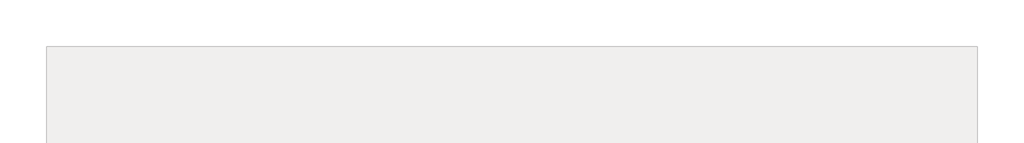
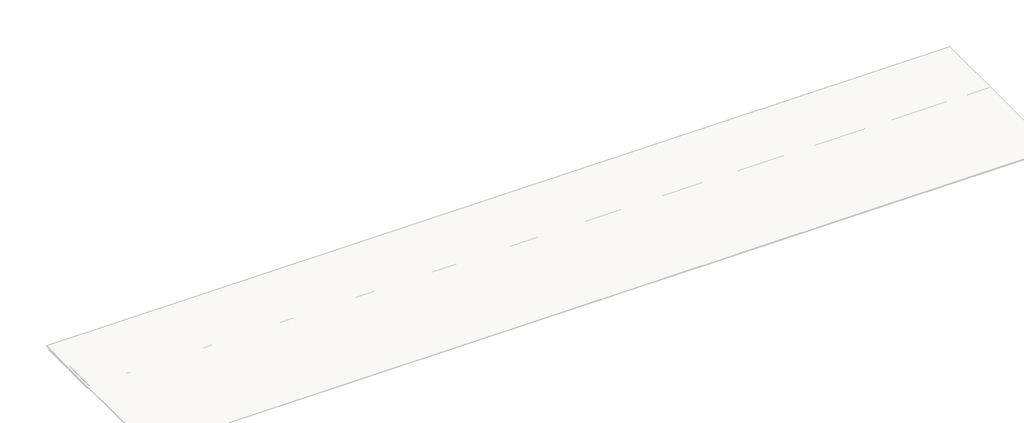
# One storey, part 4 of 4: 69 beams.
"""IFC4 building model written with IfcOpenShell, lengths in millimetres."""

from ifc_helpers import new_model, si_unit, frame, origin, place, context, project, spatial, polyline, outline, extrude, faceted_brep, element, save

model = new_model("IFC4")

# Units and contexts
model_context = context("Model", 3, world=origin())
ifc_project = project(units=[si_unit("LENGTHUNIT", "METRE", prefix="MILLI")], contexts=[model_context])

# Site, building, storey
site = spatial("IfcSite", under=ifc_project)
building = spatial("IfcBuilding", under=site)
storey = spatial("IfcBuildingStorey", under=building, Name="03_T.O.C_1", Elevation=6949.9618634)

# Beams
placement = place(None, origin())
element("IfcBeam", 1, ObjectType="RC Beam_Rectangular : H_SB_AR_S16_B300xH600", at=placement, inside=storey, context=model_context, shape_type="Brep", body=[
    faceted_brep([(2080.0, 99.5208589, 6349.9618634), (2080.0, 99.5208589, 6848.9618634), (1780.0, 99.5208589, 6848.9618634), (-4070.0, 99.5208589, 6848.9618634), (-4070.0, 99.5208589, 6349.9618634), (1780.0, 99.5208589, 6349.9618634), (2080.0, 399.5208589, 6349.9618634), (-4070.0, 399.5208589, 6349.9618634), (1780.0, 399.5208589, 6349.9618634), (2080.0, 399.5208589, 6848.9618634), (-4070.0, 399.5208589, 6848.9618634), (1780.0, 399.5208589, 6848.9618634)], [[[0, 1, 2, 3, 4, 5]], [[6, 0, 5, 4, 7, 8]], [[9, 6, 8, 7, 10, 11]], [[1, 9, 11, 10, 3, 2]], [[4, 3, 10, 7]], [[0, 6, 9, 1]]]),
])
element("IfcBeam", 2, ObjectType="RC Beam_Rectangular : H_SB_AR_S16_B300xH600", at=placement, inside=storey, context=model_context, shape_type="Brep", body=[
    faceted_brep([(10280.0, 99.5208589, 6349.9618634), (10280.0, 99.5208589, 6848.9618634), (9980.0, 99.5208589, 6848.9618634), (2080.0, 99.5208589, 6848.9618634), (2080.0, 99.5208589, 6349.9618634), (9980.0, 99.5208589, 6349.9618634), (10280.0, 399.5208589, 6349.9618634), (2080.0, 399.5208589, 6349.9618634), (9980.0, 399.5208589, 6349.9618634), (10280.0, 399.5208589, 6848.9618634), (2080.0, 399.5208589, 6848.9618634), (9980.0, 399.5208589, 6848.9618634)], [[[0, 1, 2, 3, 4, 5]], [[6, 0, 5, 4, 7, 8]], [[9, 6, 8, 7, 10, 11]], [[1, 9, 11, 10, 3, 2]], [[0, 6, 9, 1]], [[4, 3, 10, 7]]]),
])
element("IfcBeam", 3, ObjectType="RC Beam_Rectangular : H_SB_AR_S16_B300xH600", at=placement, inside=storey, context=model_context, shape_type="Brep", body=[
    faceted_brep([(18480.0, 99.5208589, 6349.9618634), (18480.0, 99.5208589, 6848.9618634), (18180.0, 99.5208589, 6848.9618634), (10280.0, 99.5208589, 6848.9618634), (10280.0, 99.5208589, 6349.9618634), (18180.0, 99.5208589, 6349.9618634), (18480.0, 399.5208589, 6349.9618634), (10280.0, 399.5208589, 6349.9618634), (18180.0, 399.5208589, 6349.9618634), (18480.0, 399.5208589, 6848.9618634), (10280.0, 399.5208589, 6848.9618634), (18180.0, 399.5208589, 6848.9618634)], [[[0, 1, 2, 3, 4, 5]], [[6, 0, 5, 4, 7, 8]], [[9, 6, 8, 7, 10, 11]], [[1, 9, 11, 10, 3, 2]], [[0, 6, 9, 1]], [[4, 3, 10, 7]]]),
])
element("IfcBeam", 4, ObjectType="RC Beam_Rectangular : H_SB_AR_S16_B300xH600", at=placement, inside=storey, context=model_context, shape_type="Brep", body=[
    faceted_brep([(26680.0, 99.5208589, 6349.9618634), (26680.0, 99.5208589, 6848.9618634), (26380.0, 99.5208589, 6848.9618634), (18480.0, 99.5208589, 6848.9618634), (18480.0, 99.5208589, 6349.9618634), (26380.0, 99.5208589, 6349.9618634), (26680.0, 399.5208589, 6349.9618634), (18480.0, 399.5208589, 6349.9618634), (26380.0, 399.5208589, 6349.9618634), (26680.0, 399.5208589, 6848.9618634), (18480.0, 399.5208589, 6848.9618634), (26380.0, 399.5208589, 6848.9618634)], [[[0, 1, 2, 3, 4, 5]], [[6, 0, 5, 4, 7, 8]], [[9, 6, 8, 7, 10, 11]], [[1, 9, 11, 10, 3, 2]], [[0, 6, 9, 1]], [[4, 3, 10, 7]]]),
])
element("IfcBeam", 5, ObjectType="RC Beam_Rectangular : H_SB_AR_S16_B300xH600", at=placement, inside=storey, context=model_context, shape_type="SweptSolid", body=[
    extrude(outline(polyline([(26680.0, 99.5208589), (26680.0, 399.5208589), (34430.0, 399.5208589), (34430.0, 99.5208589), (26680.0, 99.5208589)])), frame((0.0, 0.0, 6349.9618634), z_axis=(0.0, 0.0, 1.0), x_axis=(1.0, 0.0, 0.0)), (0.0, 0.0, 1.0), 499.0),
])
element("IfcBeam", 6, ObjectType="RC Beam_Rectangular : H_SB_AR_S16_B300xH600", at=placement, inside=storey, context=model_context, shape_type="Brep", body=[
    faceted_brep([(35630.0, 99.5208589, 6349.9618634), (35630.0, 99.5208589, 6848.9618634), (35330.0, 99.5208589, 6848.9618634), (35030.0, 99.5208589, 6848.9618634), (35030.0, 99.5208589, 6349.9618634), (35330.0, 99.5208589, 6349.9618634), (35630.0, 399.5208589, 6349.9618634), (35030.0, 399.5208589, 6349.9618634), (35330.0, 399.5208589, 6349.9618634), (35630.0, 399.5208589, 6848.9618634), (35030.0, 399.5208589, 6848.9618634), (35330.0, 399.5208589, 6848.9618634)], [[[0, 1, 2, 3, 4, 5]], [[6, 0, 5, 4, 7, 8]], [[9, 6, 8, 7, 10, 11]], [[1, 9, 11, 10, 3, 2]], [[4, 3, 10, 7]], [[0, 6, 9, 1]]]),
])
element("IfcBeam", 7, ObjectType="RC Beam_Rectangular : H_SB_AR_S16_B300xH600", at=placement, inside=storey, context=model_context, shape_type="Brep", body=[
    faceted_brep([(43830.0, 99.5208589, 6349.9618634), (43830.0, 99.5208589, 6848.9618634), (43530.0, 99.5208589, 6848.9618634), (35630.0, 99.5208589, 6848.9618634), (35630.0, 99.5208589, 6349.9618634), (43530.0, 99.5208589, 6349.9618634), (43830.0, 399.5208589, 6349.9618634), (35630.0, 399.5208589, 6349.9618634), (43530.0, 399.5208589, 6349.9618634), (43830.0, 399.5208589, 6848.9618634), (35630.0, 399.5208589, 6848.9618634), (43530.0, 399.5208589, 6848.9618634)], [[[0, 1, 2, 3, 4, 5]], [[6, 0, 5, 4, 7, 8]], [[9, 6, 8, 7, 10, 11]], [[1, 9, 11, 10, 3, 2]], [[4, 3, 10, 7]], [[0, 6, 9, 1]]]),
])
element("IfcBeam", 8, ObjectType="RC Beam_Rectangular : H_SB_AR_S16_B300xH600", at=placement, inside=storey, context=model_context, shape_type="Brep", body=[
    faceted_brep([(52030.0, 99.5208589, 6349.9618634), (52030.0, 99.5208589, 6848.9618634), (51730.0, 99.5208589, 6848.9618634), (43830.0, 99.5208589, 6848.9618634), (43830.0, 99.5208589, 6349.9618634), (51730.0, 99.5208589, 6349.9618634), (52030.0, 399.5208589, 6349.9618634), (43830.0, 399.5208589, 6349.9618634), (51730.0, 399.5208589, 6349.9618634), (52030.0, 399.5208589, 6848.9618634), (43830.0, 399.5208589, 6848.9618634), (51730.0, 399.5208589, 6848.9618634)], [[[0, 1, 2, 3, 4, 5]], [[6, 0, 5, 4, 7, 8]], [[9, 6, 8, 7, 10, 11]], [[1, 9, 11, 10, 3, 2]], [[4, 3, 10, 7]], [[0, 6, 9, 1]]]),
])
element("IfcBeam", 9, ObjectType="RC Beam_Rectangular : H_SB_AR_S16_B300xH600", at=placement, inside=storey, context=model_context, shape_type="Brep", body=[
    faceted_brep([(60230.0, 99.5208589, 6349.9618634), (60230.0, 99.5208589, 6848.9618634), (59930.0, 99.5208589, 6848.9618634), (52030.0, 99.5208589, 6848.9618634), (52030.0, 99.5208589, 6349.9618634), (59930.0, 99.5208589, 6349.9618634), (60230.0, 399.5208589, 6349.9618634), (52030.0, 399.5208589, 6349.9618634), (59930.0, 399.5208589, 6349.9618634), (60230.0, 399.5208589, 6848.9618634), (52030.0, 399.5208589, 6848.9618634), (59930.0, 399.5208589, 6848.9618634)], [[[0, 1, 2, 3, 4, 5]], [[6, 0, 5, 4, 7, 8]], [[9, 6, 8, 7, 10, 11]], [[1, 9, 11, 10, 3, 2]], [[0, 6, 9, 1]], [[4, 3, 10, 7]]]),
])
element("IfcBeam", 10, ObjectType="RC Beam_Rectangular : H_SB_AR_S16_B300xH600", at=placement, inside=storey, context=model_context, shape_type="Brep", body=[
    faceted_brep([(68430.0, 99.5208589, 6349.9618634), (68430.0, 99.5208589, 6848.9618634), (68130.0, 99.5208589, 6848.9618634), (60230.0, 99.5208589, 6848.9618634), (60230.0, 99.5208589, 6349.9618634), (68130.0, 99.5208589, 6349.9618634), (68430.0, 399.5208589, 6349.9618634), (60230.0, 399.5208589, 6349.9618634), (68130.0, 399.5208589, 6349.9618634), (68430.0, 399.5208589, 6848.9618634), (60230.0, 399.5208589, 6848.9618634), (68130.0, 399.5208589, 6848.9618634)], [[[0, 1, 2, 3, 4, 5]], [[6, 0, 5, 4, 7, 8]], [[9, 6, 8, 7, 10, 11]], [[1, 9, 11, 10, 3, 2]], [[4, 3, 10, 7]], [[0, 6, 9, 1]]]),
])
element("IfcBeam", 11, ObjectType="RC Beam_Rectangular : H_SB_AR_S16_B300xH600", at=placement, inside=storey, context=model_context, shape_type="Brep", body=[
    faceted_brep([(76630.0, 99.5208589, 6349.9618634), (76630.0, 99.5208589, 6848.9618634), (76330.0, 99.5208589, 6848.9618634), (68430.0, 99.5208589, 6848.9618634), (68430.0, 99.5208589, 6349.9618634), (76330.0, 99.5208589, 6349.9618634), (76630.0, 399.5208589, 6349.9618634), (68430.0, 399.5208589, 6349.9618634), (76330.0, 399.5208589, 6349.9618634), (76630.0, 399.5208589, 6848.9618634), (68430.0, 399.5208589, 6848.9618634), (76330.0, 399.5208589, 6848.9618634)], [[[0, 1, 2, 3, 4, 5]], [[6, 0, 5, 4, 7, 8]], [[9, 6, 8, 7, 10, 11]], [[1, 9, 11, 10, 3, 2]], [[0, 6, 9, 1]], [[4, 3, 10, 7]]]),
])
element("IfcBeam", 12, ObjectType="RC Beam_Rectangular : H_SB_AR_S16_B300xH600", at=placement, inside=storey, context=model_context, shape_type="Brep", body=[
    faceted_brep([(77380.0, 99.5208589, 6349.9618634), (77380.0, 99.5208589, 6848.9618634), (77080.0, 99.5208589, 6848.9618634), (76630.0, 99.5208589, 6848.9618634), (76630.0, 99.5208589, 6349.9618634), (77080.0, 99.5208589, 6349.9618634), (77380.0, 399.5208589, 6349.9618634), (76630.0, 399.5208589, 6349.9618634), (77080.0, 399.5208589, 6349.9618634), (77380.0, 399.5208589, 6848.9618634), (76630.0, 399.5208589, 6848.9618634), (77080.0, 399.5208589, 6848.9618634)], [[[0, 1, 2, 3, 4, 5]], [[6, 0, 5, 4, 7, 8]], [[9, 6, 8, 7, 10, 11]], [[1, 9, 11, 10, 3, 2]], [[0, 6, 9, 1]], [[4, 3, 10, 7]]]),
])
element("IfcBeam", 13, ObjectType="RC Beam_Rectangular : H_SB_AR_S16_B300xH600", at=placement, inside=storey, context=model_context, shape_type="Brep", body=[
    faceted_brep([(85580.0, 99.5208589, 6349.9618634), (85580.0, 99.5208589, 6848.9618634), (85280.0, 99.5208589, 6848.9618634), (77380.0, 99.5208589, 6848.9618634), (77380.0, 99.5208589, 6349.9618634), (85280.0, 99.5208589, 6349.9618634), (85580.0, 399.5208589, 6349.9618634), (77380.0, 399.5208589, 6349.9618634), (85280.0, 399.5208589, 6349.9618634), (85580.0, 399.5208589, 6848.9618634), (77380.0, 399.5208589, 6848.9618634), (85280.0, 399.5208589, 6848.9618634)], [[[0, 1, 2, 3, 4, 5]], [[6, 0, 5, 4, 7, 8]], [[9, 6, 8, 7, 10, 11]], [[1, 9, 11, 10, 3, 2]], [[0, 6, 9, 1]], [[4, 3, 10, 7]]]),
])
element("IfcBeam", 14, ObjectType="RC Beam_Rectangular : H_SB_AR_S16_B300xH600", at=placement, inside=storey, context=model_context, shape_type="Brep", body=[
    faceted_brep([(93780.0, 99.5208589, 6349.9618634), (93780.0, 99.5208589, 6848.9618634), (93480.0, 99.5208589, 6848.9618634), (85580.0, 99.5208589, 6848.9618634), (85580.0, 99.5208589, 6349.9618634), (93480.0, 99.5208589, 6349.9618634), (93780.0, 399.5208589, 6349.9618634), (85580.0, 399.5208589, 6349.9618634), (93480.0, 399.5208589, 6349.9618634), (93780.0, 399.5208589, 6848.9618634), (85580.0, 399.5208589, 6848.9618634), (93480.0, 399.5208589, 6848.9618634)], [[[0, 1, 2, 3, 4, 5]], [[6, 0, 5, 4, 7, 8]], [[9, 6, 8, 7, 10, 11]], [[1, 9, 11, 10, 3, 2]], [[0, 6, 9, 1]], [[4, 3, 10, 7]]]),
])
element("IfcBeam", 15, ObjectType="RC Beam_Rectangular : H_SB_AR_S16_B300xH600", at=placement, inside=storey, context=model_context, shape_type="Brep", body=[
    faceted_brep([(101980.0, 99.5208589, 6349.9618634), (101980.0, 99.5208589, 6848.9618634), (101680.0, 99.5208589, 6848.9618634), (93780.0, 99.5208589, 6848.9618634), (93780.0, 99.5208589, 6349.9618634), (101680.0, 99.5208589, 6349.9618634), (101980.0, 399.5208589, 6349.9618634), (93780.0, 399.5208589, 6349.9618634), (101680.0, 399.5208589, 6349.9618634), (101980.0, 399.5208589, 6848.9618634), (93780.0, 399.5208589, 6848.9618634), (101680.0, 399.5208589, 6848.9618634)], [[[0, 1, 2, 3, 4, 5]], [[6, 0, 5, 4, 7, 8]], [[9, 6, 8, 7, 10, 11]], [[1, 9, 11, 10, 3, 2]], [[0, 6, 9, 1]], [[4, 3, 10, 7]]]),
])
element("IfcBeam", 16, ObjectType="RC Beam_Rectangular : H_SB_AR_S16_B300xH600", at=placement, inside=storey, context=model_context, shape_type="SweptSolid", body=[
    extrude(outline(polyline([(101980.0, 99.5208589), (101980.0, 399.5208589), (109730.0, 399.5208589), (109730.0, 99.5208589), (101980.0, 99.5208589)])), frame((0.0, 0.0, 6349.9618634), z_axis=(0.0, 0.0, 1.0), x_axis=(1.0, 0.0, 0.0)), (0.0, 0.0, 1.0), 499.0),
])
element("IfcBeam", 17, ObjectType="RC Beam_Rectangular : H_SB_AR_S16_B300xH600", at=placement, inside=storey, context=model_context, shape_type="SweptSolid", body=[
    extrude(outline(polyline([(110330.0, 99.5208589), (110330.0, 399.5208589), (110480.0, 399.5208589), (110480.0, 99.5208589), (110330.0, 99.5208589)])), frame((0.0, 0.0, 6349.9618634), z_axis=(0.0, 0.0, 1.0), x_axis=(1.0, 0.0, 0.0)), (0.0, 0.0, 1.0), 499.0),
])
element("IfcBeam", 18, ObjectType="RC Beam_Rectangular : H_SB_AR_S16_B300xH600", at=placement, inside=storey, context=model_context, shape_type="SweptSolid", body=[
    extrude(outline(polyline([(111080.0, 99.5208589), (111080.0, 399.5208589), (118680.0, 399.5208589), (118680.0, 99.5208589), (111080.0, 99.5208589)])), frame((0.0, 0.0, 6349.9618634), z_axis=(0.0, 0.0, 1.0), x_axis=(1.0, 0.0, 0.0)), (0.0, 0.0, 1.0), 499.0),
])
element("IfcBeam", 19, ObjectType="RC Beam_Rectangular : H_SB_AR_S16_B300xH600", at=placement, inside=storey, context=model_context, shape_type="SweptSolid", body=[
    extrude(outline(polyline([(119280.0, 99.5208589), (119280.0, 399.5208589), (126880.0, 399.5208589), (126880.0, 99.5208589), (119280.0, 99.5208589)])), frame((0.0, 0.0, 6349.9618634), z_axis=(0.0, 0.0, 1.0), x_axis=(1.0, 0.0, 0.0)), (0.0, 0.0, 1.0), 499.0),
])
element("IfcBeam", 20, ObjectType="RC Beam_Rectangular : H_SB_AR_S16_B300xH600", at=placement, inside=storey, context=model_context, shape_type="SweptSolid", body=[
    extrude(outline(polyline([(127480.0, 99.5208589), (127480.0, 399.5208589), (135080.0, 399.5208589), (135080.0, 99.5208589), (127480.0, 99.5208589)])), frame((0.0, 0.0, 6349.9618634), z_axis=(0.0, 0.0, 1.0), x_axis=(1.0, 0.0, 0.0)), (0.0, 0.0, 1.0), 499.0),
])
element("IfcBeam", 21, ObjectType="RC Beam_Rectangular : H_SB_AR_S16_B300xH600", at=placement, inside=storey, context=model_context, shape_type="SweptSolid", body=[
    extrude(outline(polyline([(135680.0, 99.5208589), (135680.0, 399.5208589), (143280.0, 399.5208589), (143280.0, 99.5208589), (135680.0, 99.5208589)])), frame((0.0, 0.0, 6349.9618634), z_axis=(0.0, 0.0, 1.0), x_axis=(1.0, 0.0, 0.0)), (0.0, 0.0, 1.0), 499.0),
])
element("IfcBeam", 22, ObjectType="RC Beam_Rectangular : H_SB_AR_S16_B300xH600", at=placement, inside=storey, context=model_context, shape_type="SweptSolid", body=[
    extrude(outline(polyline([(143880.0, 99.5208589), (143880.0, 399.5208589), (151480.0, 399.5208589), (151480.0, 99.5208589), (143880.0, 99.5208589)])), frame((0.0, 0.0, 6349.9618634), z_axis=(0.0, 0.0, 1.0), x_axis=(1.0, 0.0, 0.0)), (0.0, 0.0, 1.0), 499.0),
])
element("IfcBeam", 23, ObjectType="RC Beam_Rectangular : H_SB_AR_S16_B300xH600", at=placement, inside=storey, context=model_context, shape_type="SweptSolid", body=[
    extrude(outline(polyline([(152080.0, 99.5208589), (152080.0, 399.5208589), (157830.0, 399.5208589), (157830.0, 99.5208589), (152080.0, 99.5208589)])), frame((0.0, 0.0, 6349.9618634), z_axis=(0.0, 0.0, 1.0), x_axis=(1.0, 0.0, 0.0)), (0.0, 0.0, 1.0), 499.0),
])
element("IfcBeam", 24, ObjectType="RC Beam_Rectangular : H_SB_AR_S16_B300xH600", at=placement, inside=storey, context=model_context, shape_type="SweptSolid", body=[
    extrude(outline(polyline([(-4070.0, 6349.5208589), (-4070.0, 6649.5208589), (1630.0, 6649.5208589), (1630.0, 6349.5208589), (-4070.0, 6349.5208589)])), frame((0.0, 0.0, 6349.9618634), z_axis=(0.0, 0.0, 1.0), x_axis=(1.0, 0.0, 0.0)), (0.0, 0.0, 1.0), 499.0),
])
element("IfcBeam", 25, ObjectType="RC Beam_Rectangular : H_SB_AR_S16_B300xH600", at=placement, inside=storey, context=model_context, shape_type="SweptSolid", body=[
    extrude(outline(polyline([(2230.0, 6349.5208589), (2230.0, 6649.5208589), (9830.0, 6649.5208589), (9830.0, 6349.5208589), (2230.0, 6349.5208589)])), frame((0.0, 0.0, 6349.9618634), z_axis=(0.0, 0.0, 1.0), x_axis=(1.0, 0.0, 0.0)), (0.0, 0.0, 1.0), 499.0),
])
element("IfcBeam", 26, ObjectType="RC Beam_Rectangular : H_SB_AR_S16_B300xH600", at=placement, inside=storey, context=model_context, shape_type="SweptSolid", body=[
    extrude(outline(polyline([(10430.0, 6349.5208589), (10430.0, 6649.5208589), (18030.0, 6649.5208589), (18030.0, 6349.5208589), (10430.0, 6349.5208589)])), frame((0.0, 0.0, 6349.9618634), z_axis=(0.0, 0.0, 1.0), x_axis=(1.0, 0.0, 0.0)), (0.0, 0.0, 1.0), 499.0),
])
element("IfcBeam", 27, ObjectType="RC Beam_Rectangular : H_SB_AR_S16_B300xH600", at=placement, inside=storey, context=model_context, shape_type="SweptSolid", body=[
    extrude(outline(polyline([(18630.0, 6349.5208589), (18630.0, 6649.5208589), (26230.0, 6649.5208589), (26230.0, 6349.5208589), (18630.0, 6349.5208589)])), frame((0.0, 0.0, 6349.9618634), z_axis=(0.0, 0.0, 1.0), x_axis=(1.0, 0.0, 0.0)), (0.0, 0.0, 1.0), 499.0),
])
element("IfcBeam", 28, ObjectType="RC Beam_Rectangular : H_SB_AR_S16_B300xH600", at=placement, inside=storey, context=model_context, shape_type="SweptSolid", body=[
    extrude(outline(polyline([(26830.0, 6349.5208589), (26830.0, 6649.5208589), (34430.0, 6649.5208589), (34430.0, 6349.5208589), (26830.0, 6349.5208589)])), frame((0.0, 0.0, 6349.9618634), z_axis=(0.0, 0.0, 1.0), x_axis=(1.0, 0.0, 0.0)), (0.0, 0.0, 1.0), 499.0),
])
element("IfcBeam", 29, ObjectType="RC Beam_Rectangular : H_SB_AR_S16_B300xH600", at=placement, inside=storey, context=model_context, shape_type="SweptSolid", body=[
    extrude(outline(polyline([(35030.0, 6349.5208589), (35030.0, 6649.5208589), (35180.0, 6649.5208589), (35180.0, 6349.5208589), (35030.0, 6349.5208589)])), frame((0.0, 0.0, 6349.9618634), z_axis=(0.0, 0.0, 1.0), x_axis=(1.0, 0.0, 0.0)), (0.0, 0.0, 1.0), 499.0),
])
element("IfcBeam", 30, ObjectType="RC Beam_Rectangular : H_SB_AR_S16_B300xH600", at=placement, inside=storey, context=model_context, shape_type="SweptSolid", body=[
    extrude(outline(polyline([(35780.0, 6349.5208589), (35780.0, 6649.5208589), (43380.0, 6649.5208589), (43380.0, 6349.5208589), (35780.0, 6349.5208589)])), frame((0.0, 0.0, 6349.9618634), z_axis=(0.0, 0.0, 1.0), x_axis=(1.0, 0.0, 0.0)), (0.0, 0.0, 1.0), 499.0),
])
element("IfcBeam", 31, ObjectType="RC Beam_Rectangular : H_SB_AR_S16_B300xH600", at=placement, inside=storey, context=model_context, shape_type="SweptSolid", body=[
    extrude(outline(polyline([(43980.0, 6349.5208589), (43980.0, 6649.5208589), (51580.0, 6649.5208589), (51580.0, 6349.5208589), (43980.0, 6349.5208589)])), frame((0.0, 0.0, 6349.9618634), z_axis=(0.0, 0.0, 1.0), x_axis=(1.0, 0.0, 0.0)), (0.0, 0.0, 1.0), 499.0),
])
element("IfcBeam", 32, ObjectType="RC Beam_Rectangular : H_SB_AR_S16_B300xH600", at=placement, inside=storey, context=model_context, shape_type="SweptSolid", body=[
    extrude(outline(polyline([(52180.0, 6349.5208589), (52180.0, 6649.5208589), (59780.0, 6649.5208589), (59780.0, 6349.5208589), (52180.0, 6349.5208589)])), frame((0.0, 0.0, 6349.9618634), z_axis=(0.0, 0.0, 1.0), x_axis=(1.0, 0.0, 0.0)), (0.0, 0.0, 1.0), 499.0),
])
element("IfcBeam", 33, ObjectType="RC Beam_Rectangular : H_SB_AR_S16_B300xH600", at=placement, inside=storey, context=model_context, shape_type="SweptSolid", body=[
    extrude(outline(polyline([(60380.0, 6349.5208589), (60380.0, 6649.5208589), (67980.0, 6649.5208589), (67980.0, 6349.5208589), (60380.0, 6349.5208589)])), frame((0.0, 0.0, 6349.9618634), z_axis=(0.0, 0.0, 1.0), x_axis=(1.0, 0.0, 0.0)), (0.0, 0.0, 1.0), 499.0),
])
element("IfcBeam", 34, ObjectType="RC Beam_Rectangular : H_SB_AR_S16_B300xH600", at=placement, inside=storey, context=model_context, shape_type="SweptSolid", body=[
    extrude(outline(polyline([(68580.0, 6349.5208589), (68580.0, 6649.5208589), (76180.0, 6649.5208589), (76180.0, 6349.5208589), (68580.0, 6349.5208589)])), frame((0.0, 0.0, 6349.9618634), z_axis=(0.0, 0.0, 1.0), x_axis=(1.0, 0.0, 0.0)), (0.0, 0.0, 1.0), 499.0),
])
element("IfcBeam", 35, ObjectType="RC Beam_Rectangular : H_SB_AR_S16_B300xH600", at=placement, inside=storey, context=model_context, shape_type="SweptSolid", body=[
    extrude(outline(polyline([(76780.0, 6349.5208589), (76780.0, 6649.5208589), (76930.0, 6649.5208589), (76930.0, 6349.5208589), (76780.0, 6349.5208589)])), frame((0.0, 0.0, 6349.9618634), z_axis=(0.0, 0.0, 1.0), x_axis=(1.0, 0.0, 0.0)), (0.0, 0.0, 1.0), 499.0),
])
element("IfcBeam", 36, ObjectType="RC Beam_Rectangular : H_SB_AR_S16_B300xH600", at=placement, inside=storey, context=model_context, shape_type="SweptSolid", body=[
    extrude(outline(polyline([(77530.0, 6349.5208589), (77530.0, 6649.5208589), (85130.0, 6649.5208589), (85130.0, 6349.5208589), (77530.0, 6349.5208589)])), frame((0.0, 0.0, 6349.9618634), z_axis=(0.0, 0.0, 1.0), x_axis=(1.0, 0.0, 0.0)), (0.0, 0.0, 1.0), 499.0),
])
element("IfcBeam", 37, ObjectType="RC Beam_Rectangular : H_SB_AR_S16_B300xH600", at=placement, inside=storey, context=model_context, shape_type="SweptSolid", body=[
    extrude(outline(polyline([(85730.0, 6349.5208589), (85730.0, 6649.5208589), (93330.0, 6649.5208589), (93330.0, 6349.5208589), (85730.0, 6349.5208589)])), frame((0.0, 0.0, 6349.9618634), z_axis=(0.0, 0.0, 1.0), x_axis=(1.0, 0.0, 0.0)), (0.0, 0.0, 1.0), 499.0),
])
element("IfcBeam", 38, ObjectType="RC Beam_Rectangular : H_SB_AR_S16_B300xH600", at=placement, inside=storey, context=model_context, shape_type="SweptSolid", body=[
    extrude(outline(polyline([(93930.0, 6349.5208589), (93930.0, 6649.5208589), (101530.0, 6649.5208589), (101530.0, 6349.5208589), (93930.0, 6349.5208589)])), frame((0.0, 0.0, 6349.9618634), z_axis=(0.0, 0.0, 1.0), x_axis=(1.0, 0.0, 0.0)), (0.0, 0.0, 1.0), 499.0),
])
element("IfcBeam", 39, ObjectType="RC Beam_Rectangular : H_SB_AR_S16_B300xH600", at=placement, inside=storey, context=model_context, shape_type="SweptSolid", body=[
    extrude(outline(polyline([(102130.0, 6349.5208589), (102130.0, 6649.5208589), (109730.0, 6649.5208589), (109730.0, 6349.5208589), (102130.0, 6349.5208589)])), frame((0.0, 0.0, 6349.9618634), z_axis=(0.0, 0.0, 1.0), x_axis=(1.0, 0.0, 0.0)), (0.0, 0.0, 1.0), 499.0),
])
element("IfcBeam", 40, ObjectType="RC Beam_Rectangular : H_SB_AR_S16_B300xH600", at=placement, inside=storey, context=model_context, shape_type="SweptSolid", body=[
    extrude(outline(polyline([(110330.0, 6349.5208589), (110330.0, 6649.5208589), (110480.0, 6649.5208589), (110480.0, 6349.5208589), (110330.0, 6349.5208589)])), frame((0.0, 0.0, 6349.9618634), z_axis=(0.0, 0.0, 1.0), x_axis=(1.0, 0.0, 0.0)), (0.0, 0.0, 1.0), 499.0),
])
element("IfcBeam", 41, ObjectType="RC Beam_Rectangular : H_SB_AR_S16_B300xH600", at=placement, inside=storey, context=model_context, shape_type="SweptSolid", body=[
    extrude(outline(polyline([(111080.0, 6349.5208589), (111080.0, 6649.5208589), (118680.0, 6649.5208589), (118680.0, 6349.5208589), (111080.0, 6349.5208589)])), frame((0.0, 0.0, 6349.9618634), z_axis=(0.0, 0.0, 1.0), x_axis=(1.0, 0.0, 0.0)), (0.0, 0.0, 1.0), 499.0),
])
element("IfcBeam", 42, ObjectType="RC Beam_Rectangular : H_SB_AR_S16_B300xH600", at=placement, inside=storey, context=model_context, shape_type="SweptSolid", body=[
    extrude(outline(polyline([(119280.0, 6349.5208589), (119280.0, 6649.5208589), (126880.0, 6649.5208589), (126880.0, 6349.5208589), (119280.0, 6349.5208589)])), frame((0.0, 0.0, 6349.9618634), z_axis=(0.0, 0.0, 1.0), x_axis=(1.0, 0.0, 0.0)), (0.0, 0.0, 1.0), 499.0),
])
element("IfcBeam", 43, ObjectType="RC Beam_Rectangular : H_SB_AR_S16_B300xH600", at=placement, inside=storey, context=model_context, shape_type="SweptSolid", body=[
    extrude(outline(polyline([(127480.0, 6349.5208589), (127480.0, 6649.5208589), (135080.0, 6649.5208589), (135080.0, 6349.5208589), (127480.0, 6349.5208589)])), frame((0.0, 0.0, 6349.9618634), z_axis=(0.0, 0.0, 1.0), x_axis=(1.0, 0.0, 0.0)), (0.0, 0.0, 1.0), 499.0),
])
element("IfcBeam", 44, ObjectType="RC Beam_Rectangular : H_SB_AR_S16_B300xH600", at=placement, inside=storey, context=model_context, shape_type="SweptSolid", body=[
    extrude(outline(polyline([(135680.0, 6349.5208589), (135680.0, 6649.5208589), (143280.0, 6649.5208589), (143280.0, 6349.5208589), (135680.0, 6349.5208589)])), frame((0.0, 0.0, 6349.9618634), z_axis=(0.0, 0.0, 1.0), x_axis=(1.0, 0.0, 0.0)), (0.0, 0.0, 1.0), 499.0),
])
element("IfcBeam", 45, ObjectType="RC Beam_Rectangular : H_SB_AR_S16_B300xH600", at=placement, inside=storey, context=model_context, shape_type="SweptSolid", body=[
    extrude(outline(polyline([(143880.0, 6349.5208589), (143880.0, 6649.5208589), (151480.0, 6649.5208589), (151480.0, 6349.5208589), (143880.0, 6349.5208589)])), frame((0.0, 0.0, 6349.9618634), z_axis=(0.0, 0.0, 1.0), x_axis=(1.0, 0.0, 0.0)), (0.0, 0.0, 1.0), 499.0),
])
element("IfcBeam", 46, ObjectType="RC Beam_Rectangular : H_SB_AR_S16_B300xH600", at=placement, inside=storey, context=model_context, shape_type="SweptSolid", body=[
    extrude(outline(polyline([(152080.0, 6349.5208589), (152080.0, 6649.5208589), (157830.0, 6649.5208589), (157830.0, 6349.5208589), (152080.0, 6349.5208589)])), frame((0.0, 0.0, 6349.9618634), z_axis=(0.0, 0.0, 1.0), x_axis=(1.0, 0.0, 0.0)), (0.0, 0.0, 1.0), 499.0),
])
element("IfcBeam", 47, ObjectType="RC Beam_Rectangular : H_SB_AR_S16_B300xH600", at=placement, inside=storey, context=model_context, shape_type="SweptSolid", body=[
    extrude(outline(polyline([(2080.0, 399.5208589), (1780.0, 399.5208589), (1780.0, 6199.5208589), (2080.0, 6199.5208589), (2080.0, 399.5208589)])), frame((0.0, 0.0, 6349.9618634), z_axis=(0.0, 0.0, 1.0), x_axis=(1.0, 0.0, 0.0)), (0.0, 0.0, 1.0), 499.0),
])
element("IfcBeam", 48, ObjectType="RC Beam_Rectangular : H_SB_AR_S16_B300xH600", at=placement, inside=storey, context=model_context, shape_type="SweptSolid", body=[
    extrude(outline(polyline([(10280.0, 399.5208589), (9980.0, 399.5208589), (9980.0, 6199.5208589), (10280.0, 6199.5208589), (10280.0, 399.5208589)])), frame((0.0, 0.0, 6349.9618634), z_axis=(0.0, 0.0, 1.0), x_axis=(1.0, 0.0, 0.0)), (0.0, 0.0, 1.0), 499.0),
])
element("IfcBeam", 49, ObjectType="RC Beam_Rectangular : H_SB_AR_S16_B300xH600", at=placement, inside=storey, context=model_context, shape_type="SweptSolid", body=[
    extrude(outline(polyline([(18480.0, 399.5208589), (18180.0, 399.5208589), (18180.0, 6199.5208589), (18480.0, 6199.5208589), (18480.0, 399.5208589)])), frame((0.0, 0.0, 6349.9618634), z_axis=(0.0, 0.0, 1.0), x_axis=(1.0, 0.0, 0.0)), (0.0, 0.0, 1.0), 499.0),
])
element("IfcBeam", 50, ObjectType="RC Beam_Rectangular : H_SB_AR_S16_B300xH600", at=placement, inside=storey, context=model_context, shape_type="SweptSolid", body=[
    extrude(outline(polyline([(26680.0, 399.5208589), (26380.0, 399.5208589), (26380.0, 6199.5208589), (26680.0, 6199.5208589), (26680.0, 399.5208589)])), frame((0.0, 0.0, 6349.9618634), z_axis=(0.0, 0.0, 1.0), x_axis=(1.0, 0.0, 0.0)), (0.0, 0.0, 1.0), 499.0),
])
element("IfcBeam", 51, ObjectType="RC Beam_Rectangular : H_SB_AR_S16_B300xH600", at=placement, inside=storey, context=model_context, shape_type="SweptSolid", body=[
    extrude(outline(polyline([(34880.0, 549.5208589), (34580.0, 549.5208589), (34580.0, 6199.5208589), (34880.0, 6199.5208589), (34880.0, 549.5208589)])), frame((0.0, 0.0, 6349.9618634), z_axis=(0.0, 0.0, 1.0), x_axis=(1.0, 0.0, 0.0)), (0.0, 0.0, 1.0), 499.0),
])
element("IfcBeam", 52, ObjectType="RC Beam_Rectangular : H_SB_AR_S16_B300xH600", at=placement, inside=storey, context=model_context, shape_type="SweptSolid", body=[
    extrude(outline(polyline([(35630.0, 399.5208589), (35330.0, 399.5208589), (35330.0, 6199.5208589), (35630.0, 6199.5208589), (35630.0, 399.5208589)])), frame((0.0, 0.0, 6349.9618634), z_axis=(0.0, 0.0, 1.0), x_axis=(1.0, 0.0, 0.0)), (0.0, 0.0, 1.0), 499.0),
])
element("IfcBeam", 53, ObjectType="RC Beam_Rectangular : H_SB_AR_S16_B300xH600", at=placement, inside=storey, context=model_context, shape_type="SweptSolid", body=[
    extrude(outline(polyline([(43830.0, 399.5208589), (43530.0, 399.5208589), (43530.0, 6199.5208589), (43830.0, 6199.5208589), (43830.0, 399.5208589)])), frame((0.0, 0.0, 6349.9618634), z_axis=(0.0, 0.0, 1.0), x_axis=(1.0, 0.0, 0.0)), (0.0, 0.0, 1.0), 499.0),
])
element("IfcBeam", 54, ObjectType="RC Beam_Rectangular : H_SB_AR_S16_B300xH600", at=placement, inside=storey, context=model_context, shape_type="SweptSolid", body=[
    extrude(outline(polyline([(52030.0, 399.5208589), (51730.0, 399.5208589), (51730.0, 6199.5208589), (52030.0, 6199.5208589), (52030.0, 399.5208589)])), frame((0.0, 0.0, 6349.9618634), z_axis=(0.0, 0.0, 1.0), x_axis=(1.0, 0.0, 0.0)), (0.0, 0.0, 1.0), 499.0),
])
element("IfcBeam", 55, ObjectType="RC Beam_Rectangular : H_SB_AR_S16_B300xH600", at=placement, inside=storey, context=model_context, shape_type="SweptSolid", body=[
    extrude(outline(polyline([(60230.0, 399.5208589), (59930.0, 399.5208589), (59930.0, 6199.5208589), (60230.0, 6199.5208589), (60230.0, 399.5208589)])), frame((0.0, 0.0, 6349.9618634), z_axis=(0.0, 0.0, 1.0), x_axis=(1.0, 0.0, 0.0)), (0.0, 0.0, 1.0), 499.0),
])
element("IfcBeam", 56, ObjectType="RC Beam_Rectangular : H_SB_AR_S16_B300xH600", at=placement, inside=storey, context=model_context, shape_type="SweptSolid", body=[
    extrude(outline(polyline([(68430.0, 399.5208589), (68130.0, 399.5208589), (68130.0, 6199.5208589), (68430.0, 6199.5208589), (68430.0, 399.5208589)])), frame((0.0, 0.0, 6349.9618634), z_axis=(0.0, 0.0, 1.0), x_axis=(1.0, 0.0, 0.0)), (0.0, 0.0, 1.0), 499.0),
])
element("IfcBeam", 57, ObjectType="RC Beam_Rectangular : H_SB_AR_S16_B300xH600", at=placement, inside=storey, context=model_context, shape_type="SweptSolid", body=[
    extrude(outline(polyline([(76630.0, 399.5208589), (76330.0, 399.5208589), (76330.0, 6199.5208589), (76630.0, 6199.5208589), (76630.0, 399.5208589)])), frame((0.0, 0.0, 6349.9618634), z_axis=(0.0, 0.0, 1.0), x_axis=(1.0, 0.0, 0.0)), (0.0, 0.0, 1.0), 499.0),
])
element("IfcBeam", 58, ObjectType="RC Beam_Rectangular : H_SB_AR_S16_B300xH600", at=placement, inside=storey, context=model_context, shape_type="SweptSolid", body=[
    extrude(outline(polyline([(77380.0, 399.5208589), (77080.0, 399.5208589), (77080.0, 6199.5208589), (77380.0, 6199.5208589), (77380.0, 399.5208589)])), frame((0.0, 0.0, 6349.9618634), z_axis=(0.0, 0.0, 1.0), x_axis=(1.0, 0.0, 0.0)), (0.0, 0.0, 1.0), 499.0),
])
element("IfcBeam", 59, ObjectType="RC Beam_Rectangular : H_SB_AR_S16_B300xH600", at=placement, inside=storey, context=model_context, shape_type="SweptSolid", body=[
    extrude(outline(polyline([(85580.0, 399.5208589), (85280.0, 399.5208589), (85280.0, 6199.5208589), (85580.0, 6199.5208589), (85580.0, 399.5208589)])), frame((0.0, 0.0, 6349.9618634), z_axis=(0.0, 0.0, 1.0), x_axis=(1.0, 0.0, 0.0)), (0.0, 0.0, 1.0), 499.0),
])
element("IfcBeam", 60, ObjectType="RC Beam_Rectangular : H_SB_AR_S16_B300xH600", at=placement, inside=storey, context=model_context, shape_type="SweptSolid", body=[
    extrude(outline(polyline([(93780.0, 399.5208589), (93480.0, 399.5208589), (93480.0, 6199.5208589), (93780.0, 6199.5208589), (93780.0, 399.5208589)])), frame((0.0, 0.0, 6349.9618634), z_axis=(0.0, 0.0, 1.0), x_axis=(1.0, 0.0, 0.0)), (0.0, 0.0, 1.0), 499.0),
])
element("IfcBeam", 61, ObjectType="RC Beam_Rectangular : H_SB_AR_S16_B300xH600", at=placement, inside=storey, context=model_context, shape_type="SweptSolid", body=[
    extrude(outline(polyline([(101980.0, 399.5208589), (101680.0, 399.5208589), (101680.0, 6199.5208589), (101980.0, 6199.5208589), (101980.0, 399.5208589)])), frame((0.0, 0.0, 6349.9618634), z_axis=(0.0, 0.0, 1.0), x_axis=(1.0, 0.0, 0.0)), (0.0, 0.0, 1.0), 499.0),
])
element("IfcBeam", 62, ObjectType="RC Beam_Rectangular : H_SB_AR_S16_B300xH600", at=placement, inside=storey, context=model_context, shape_type="SweptSolid", body=[
    extrude(outline(polyline([(110180.0, 549.5208589), (109880.0, 549.5208589), (109880.0, 6199.5208589), (110180.0, 6199.5208589), (110180.0, 549.5208589)])), frame((0.0, 0.0, 6349.9618634), z_axis=(0.0, 0.0, 1.0), x_axis=(1.0, 0.0, 0.0)), (0.0, 0.0, 1.0), 499.0),
])
element("IfcBeam", 63, ObjectType="RC Beam_Rectangular : H_SB_AR_S16_B300xH600", at=placement, inside=storey, context=model_context, shape_type="SweptSolid", body=[
    extrude(outline(polyline([(110930.0, 549.5208589), (110630.0, 549.5208589), (110630.0, 6199.5208589), (110930.0, 6199.5208589), (110930.0, 549.5208589)])), frame((0.0, 0.0, 6349.9618634), z_axis=(0.0, 0.0, 1.0), x_axis=(1.0, 0.0, 0.0)), (0.0, 0.0, 1.0), 499.0),
])
element("IfcBeam", 64, ObjectType="RC Beam_Rectangular : H_SB_AR_S16_B300xH600", at=placement, inside=storey, context=model_context, shape_type="SweptSolid", body=[
    extrude(outline(polyline([(119130.0, 549.5208589), (118830.0, 549.5208589), (118830.0, 6199.5208589), (119130.0, 6199.5208589), (119130.0, 549.5208589)])), frame((0.0, 0.0, 6349.9618634), z_axis=(0.0, 0.0, 1.0), x_axis=(1.0, 0.0, 0.0)), (0.0, 0.0, 1.0), 499.0),
])
element("IfcBeam", 65, ObjectType="RC Beam_Rectangular : H_SB_AR_S16_B300xH600", at=placement, inside=storey, context=model_context, shape_type="SweptSolid", body=[
    extrude(outline(polyline([(127330.0, 549.5208589), (127030.0, 549.5208589), (127030.0, 6199.5208589), (127330.0, 6199.5208589), (127330.0, 549.5208589)])), frame((0.0, 0.0, 6349.9618634), z_axis=(0.0, 0.0, 1.0), x_axis=(1.0, 0.0, 0.0)), (0.0, 0.0, 1.0), 499.0),
])
element("IfcBeam", 66, ObjectType="RC Beam_Rectangular : H_SB_AR_S16_B300xH600", at=placement, inside=storey, context=model_context, shape_type="SweptSolid", body=[
    extrude(outline(polyline([(135530.0, 549.5208589), (135230.0, 549.5208589), (135230.0, 6199.5208589), (135530.0, 6199.5208589), (135530.0, 549.5208589)])), frame((0.0, 0.0, 6349.9618634), z_axis=(0.0, 0.0, 1.0), x_axis=(1.0, 0.0, 0.0)), (0.0, 0.0, 1.0), 499.0),
])
element("IfcBeam", 67, ObjectType="RC Beam_Rectangular : H_SB_AR_S16_B300xH600", at=placement, inside=storey, context=model_context, shape_type="SweptSolid", body=[
    extrude(outline(polyline([(143730.0, 549.5208589), (143430.0, 549.5208589), (143430.0, 6199.5208589), (143730.0, 6199.5208589), (143730.0, 549.5208589)])), frame((0.0, 0.0, 6349.9618634), z_axis=(0.0, 0.0, 1.0), x_axis=(1.0, 0.0, 0.0)), (0.0, 0.0, 1.0), 499.0),
])
element("IfcBeam", 68, ObjectType="RC Beam_Rectangular : H_SB_AR_S16_B300xH600", at=placement, inside=storey, context=model_context, shape_type="SweptSolid", body=[
    extrude(outline(polyline([(151930.0, 549.5208589), (151630.0, 549.5208589), (151630.0, 6199.5208589), (151930.0, 6199.5208589), (151930.0, 549.5208589)])), frame((0.0, 0.0, 6349.9618634), z_axis=(0.0, 0.0, 1.0), x_axis=(1.0, 0.0, 0.0)), (0.0, 0.0, 1.0), 499.0),
])
element("IfcBeam", 69, ObjectType="RC Beam_Rectangular : H_SB_AR_S16_B300xH600", at=placement, inside=storey, context=model_context, shape_type="SweptSolid", body=[
    extrude(outline(polyline([(158280.0, 549.5208589), (157980.0, 549.5208589), (157980.0, 6199.5208589), (158280.0, 6199.5208589), (158280.0, 549.5208589)])), frame((0.0, 0.0, 6349.9618634), z_axis=(0.0, 0.0, 1.0), x_axis=(1.0, 0.0, 0.0)), (0.0, 0.0, 1.0), 499.0),
])

save(model, "model.ifc")

# Revit data of these elements
# Type "RC Beam_Rectangular : H_SB_AR_S16_B300xH600"
#   중앙부 하부근 = ""
#   중앙부 상부근 = ""
#   중앙부 보조근 = ""
#   중앙부 늑근 = ""
#   외단부 하부근 = ""
#   외단부 상부근 = ""
#   외단부 보조근 = ""
#   외단부 늑근 = ""
#   부호 = "TG3"
#   내단부 하부근 = ""
#   내단부 상부근 = ""
#   내단부 보조근 = ""
#   내단부 늑근 = ""
#   ALL 하부근 = "3-D20"
#   ALL 상부근 = "3-D20"
#   ALL 보조근 = ""
#   ALL 늑근 = "2-D10 @120"
#   Width = 300 mm
#   Height = 600 mm
#   Length [instance default] = 1524 mm
#   b = 300 mm
#   h = 600 mm
#   hec_material3 [instance default] = none
#   hec_material2 [instance default] = none
#   hec_material1 [instance default] = none
#   Structural Material [instance default] = none
#   Assembly Code = ""
# Elements 1, 2, 3, 4, 5, 6, 7, 8, 9, 10, 11, 12, 13, 14, 15, 16, 17, 18, 19, 20, 21, 22, 23, 24, 25, 26, 27, 28, 29, 30, 31, 32, 33, 34, 35, 36, 37, 38, 39, 40, 41, 42, 43, 44, 45, 46, 47, 48, 49, 50, 51, 52, 53, 54, 55, 56, 57, 58, 59, 60, 61, 62, 63, 64, 65, 66, 67, 68, 69 (IfcBeam, "RC Beam_Rectangular : H_SB_AR_S16_B300xH600")
#   Comments = ""
#   hec_material3 = none
#   hec_material2 = none
#   hec_material1 = none
#   Structural Material = none
#   Phase Created = New Construction
